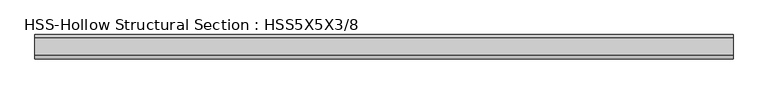
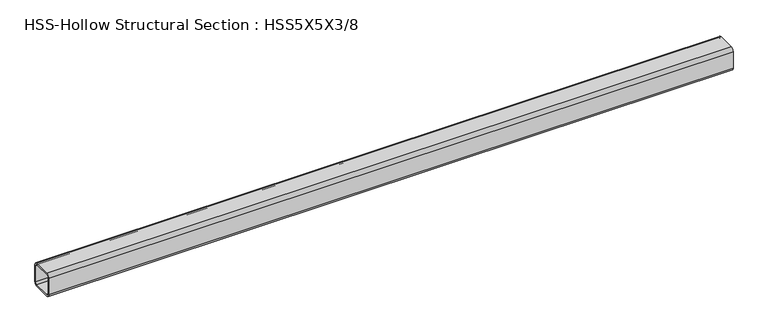
"""IFC4 building model written with IfcOpenShell, lengths in millimetres: beam geometry, HSS-Hollow Structural Section : HSS5X5X3/8."""

from ifc_helpers import new_model, si_unit, point, frame, frame_2d, origin, place, context, project, spatial, polyline, circle_curve, trimmed, segment, composite_curve, outline, extrude, source, transform, mapped, element, save


def hss_hollow_structural_section_hss5x5x3_8_b56cee5d(model_context):
    return source(origin(), model_context, "Body", "SweptSolid", [
        extrude(outline(composite_curve([segment(trimmed(circle_curve(frame_2d((-45.7708, 45.7708)), 17.7292), [point((-63.5, 45.7708))], [point((-45.7708, 63.5))], False, "CARTESIAN"), True, "CONTINUOUS"), segment(polyline([(-45.7708, 63.5), (45.7708, 63.5)]), True, "CONTINUOUS"), segment(trimmed(circle_curve(frame_2d((45.7708, 45.7708)), 17.7292), [point((45.7708, 63.5))], [point((63.5, 45.7708))], False, "CARTESIAN"), True, "CONTINUOUS"), segment(polyline([(63.5, 45.7708), (63.5, -45.7708)]), True, "CONTINUOUS"), segment(trimmed(circle_curve(frame_2d((45.7708, -45.7708)), 17.7292), [point((63.5, -45.7708))], [point((45.7708, -63.5))], False, "CARTESIAN"), True, "CONTINUOUS"), segment(polyline([(45.7708, -63.5), (-45.7708, -63.5)]), True, "CONTINUOUS"), segment(trimmed(circle_curve(frame_2d((-45.7708, -45.7708)), 17.7292), [point((-45.7708, -63.5))], [point((-63.5, -45.7708))], False, "CARTESIAN"), True, "CONTINUOUS"), segment(polyline([(-63.5, -45.7708), (-63.5, 45.7708)]), True, "CONTINUOUS")], self_intersect=False), holes=[composite_curve([segment(polyline([(45.7708, 54.6354), (-45.7708, 54.6354)]), True, "CONTINUOUS"), segment(trimmed(circle_curve(frame_2d((-45.7708, 45.7708)), 8.8646), [point((-45.7708, 54.6354))], [point((-54.6354, 45.7708))], True, "CARTESIAN"), True, "CONTINUOUS"), segment(polyline([(-54.6354, 45.7708), (-54.6354, -45.7708)]), True, "CONTINUOUS"), segment(trimmed(circle_curve(frame_2d((-45.7708, -45.7708)), 8.8646), [point((-54.6354, -45.7708))], [point((-45.7708, -54.6354))], True, "CARTESIAN"), True, "CONTINUOUS"), segment(polyline([(-45.7708, -54.6354), (45.7708, -54.6354)]), True, "CONTINUOUS"), segment(trimmed(circle_curve(frame_2d((45.7708, -45.7708)), 8.8646), [point((45.7708, -54.6354))], [point((54.6354, -45.7708))], True, "CARTESIAN"), True, "CONTINUOUS"), segment(polyline([(54.6354, -45.7708), (54.6354, 45.7708)]), True, "CONTINUOUS"), segment(trimmed(circle_curve(frame_2d((45.7708, 45.7708)), 8.8646), [point((54.6354, 45.7708))], [point((45.7708, 54.6354))], True, "CARTESIAN"), True, "CONTINUOUS")], self_intersect=False)]), frame((-1812.925, 0.0, 0.0), z_axis=(1.0, 0.0, 0.0), x_axis=(0.0, 1.0, 0.0)), (0.0, 0.0, 1.0), 3625.85),
    ])


if __name__ == "__main__":
    model = new_model("IFC4")
    model_context = context("Model", 3, world=origin())
    ifc_project = project(units=[si_unit("LENGTHUNIT", "METRE", prefix="MILLI")], contexts=[model_context])
    site = spatial("IfcSite", under=ifc_project)
    building = spatial("IfcBuilding", under=site)
    placement = place(None, origin())
    hss_hollow_structural_section_hss5x5x3_8_shape = hss_hollow_structural_section_hss5x5x3_8_b56cee5d(model_context)
    element("IfcBeam", 1, ObjectType="HSS-Hollow Structural Section : HSS5X5X3/8", at=placement, inside=building, context=model_context, shape_type="MappedRepresentation", body=[
        mapped(hss_hollow_structural_section_hss5x5x3_8_shape, transform((0.0, 0.0, 0.0), x_axis=(1.0, 0.0, 0.0), y_axis=(0.0, 1.0, 0.0), z_axis=(0.0, 0.0, 1.0))),
    ])
    save(model, "model.ifc")

# Revit data of these elements
# Type "HSS-Hollow Structural Section : HSS5X5X3/8"
#   Assembly Code = "B10"
#   Shape = "Square"
#   W = 22.3
#   Ht = 0' - 5"
#   Length [instance default] = 5' - 0"
#   b = 0' - 5"
#   kr = 0' - 0.698"
#   t = 0' - 0.349"
#   A = 0.0429167 SF
#   Structural Material [instance default] = Steel ASTM A500, Grade B, Rectangular and Square
# Element 1 (IfcBeam, "HSS-Hollow Structural Section : HSS5X5X3/8")
#   Materials on its faces: "Steel ASTM A500, Grade B, Rectangular and Square"
# Materials
#   "Steel ASTM A500, Grade B, Rectangular and Square": class "Metal", colour RGB 199 199 199, transparency 0, Description = "Carbon steel", Cost = 0
